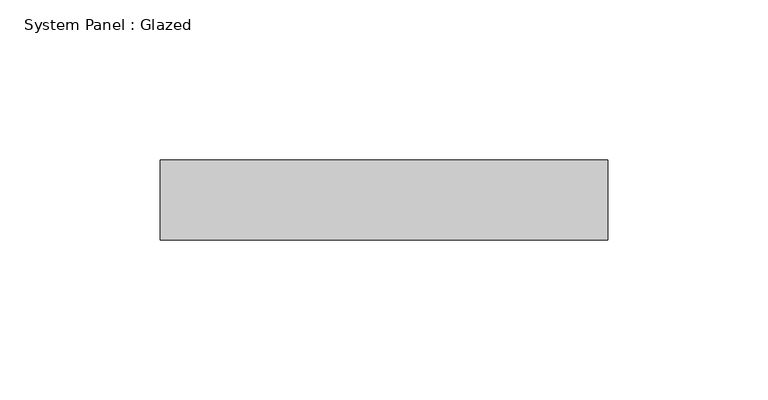
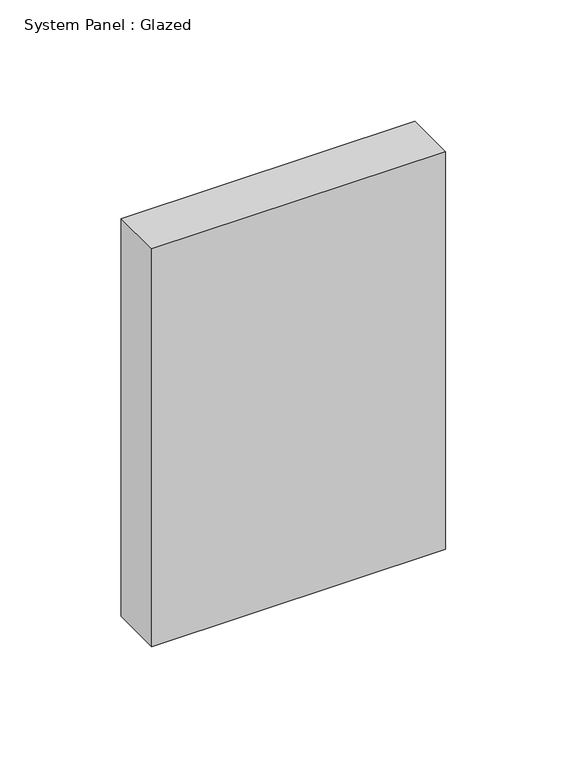
"""IFC4 building model written with IfcOpenShell, lengths in millimetres: plate geometry, System Panel : Glazed."""

from ifc_helpers import new_model, si_unit, origin, origin_with_axes, place, context, project, spatial, polyline, outline, extrude, source, transform, mapped, element, save


def system_panel_glazed_b673c039(model_context):
    return source(origin(), model_context, "Body", "SweptSolid", [
        extrude(outline(polyline([(69.8854993, 24.5), (-69.8854993, 24.5), (-69.8854993, 49.5), (69.8854993, 49.5), (69.8854993, 24.5)])), origin_with_axes(), (0.0, 0.0, 1.0), 200.0),
    ])


if __name__ == "__main__":
    model = new_model("IFC4")
    model_context = context("Model", 3, world=origin())
    ifc_project = project(units=[si_unit("LENGTHUNIT", "METRE", prefix="MILLI")], contexts=[model_context])
    site = spatial("IfcSite", under=ifc_project)
    building = spatial("IfcBuilding", under=site)
    placement = place(None, origin())
    system_panel_glazed_shape = system_panel_glazed_b673c039(model_context)
    element("IfcPlate", 1, ObjectType="System Panel : Glazed", at=placement, inside=building, context=model_context, shape_type="MappedRepresentation", body=[
        mapped(system_panel_glazed_shape, transform((0.0, 0.0, 0.0), x_axis=(1.0, 0.0, 0.0), y_axis=(0.0, 1.0, 0.0), z_axis=(0.0, 0.0, 1.0))),
    ])
    save(model, "model.ifc")

# Revit data of these elements
# Element 1 (IfcPlate, "System Panel : Glazed")
#   Materials on its faces: "Glass"
# Materials
#   "Glass": class "Glass", colour RGB 218 227 224, transparency 0.85, Description = "Soda Lime Glass", Cost = 0
